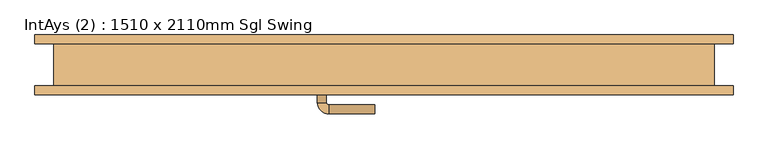
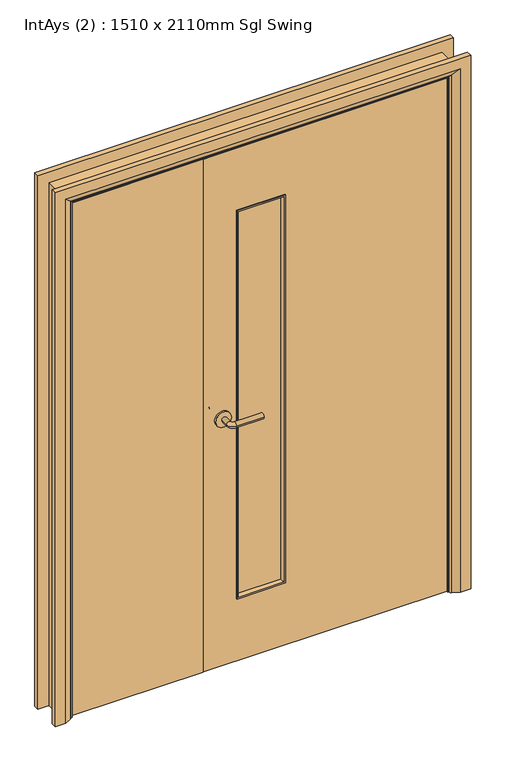
"""IFC4 building model written with IfcOpenShell, lengths in millimetres: door geometry, IntAys (2) : 1510 x 2110mm Sgl Swing."""

from ifc_helpers import new_model, si_unit, point, frame, frame_2d, origin, place, context, project, spatial, polyline, circle_curve, ellipse_curve, trimmed, segment, composite_curve, outline, extrude, faceted_brep, source, transform, mapped, element, save
from ifc_brep_helpers import plane_surface, cylinder_surface, revolved_surface, advanced_brep


def intays_2_1510_x_2110mm_sgl_swing_7badbe2f(model_context):
    return source(origin(), model_context, "Body", "SolidModel", [
        advanced_brep(
        [(88.5, -7.5, 1000.0), (108.5, -7.5, 1000.0), (88.5, 22.5, 1000.0), (108.5, 22.5, 1000.0), (113.5, 27.5, 1000.0), (113.5, 47.5, 1000.0), (218.5, 47.5, 1000.0), (218.5, 27.5, 1000.0)],
        [
            (0, 1, circle_curve(frame((98.5, -7.5, 1000.0), z_axis=(0.0, -1.0, 0.0), x_axis=(1.0, 0.0, 0.0)), 10.0)),
            (1, 0, circle_curve(frame((98.5, -7.5, 1000.0), z_axis=(0.0, -1.0, 0.0), x_axis=(1.0, 0.0, 0.0)), 10.0)),
            (0, 2),
            (2, 3, circle_curve(frame((98.5, 22.5, 1000.0), z_axis=(0.0, -1.0, 0.0), x_axis=(1.0, 0.0, 0.0)), 10.0)),
            (3, 1),
            (3, 2, circle_curve(frame((98.5, 22.5, 1000.0), z_axis=(0.0, -1.0, 0.0), x_axis=(1.0, 0.0, 0.0)), 10.0)),
            (4, 3, circle_curve(frame((113.5, 22.5, 1000.0), z_axis=(0.0, 0.0, 1.0), x_axis=(-1.0, 0.0, 0.0)), 5.0)),
            (2, 5, circle_curve(frame((113.5, 22.5, 1000.0), z_axis=(0.0, 0.0, -1.0), x_axis=(-1.0, 0.0, 0.0)), 25.0)),
            (5, 4, circle_curve(frame((113.5, 37.5, 1000.0), z_axis=(-1.0, 0.0, 0.0), x_axis=(0.0, -1.0, 0.0)), 10.0)),
            (4, 5, circle_curve(frame((113.5, 37.5, 1000.0), z_axis=(-1.0, 0.0, 0.0), x_axis=(0.0, -1.0, 0.0)), 10.0)),
            (6, 7, circle_curve(frame((218.5, 37.5, 1000.0), z_axis=(1.0, 0.0, 0.0), x_axis=(0.0, -1.0, 0.0)), 10.0)),
            (7, 6, circle_curve(frame((218.5, 37.5, 1000.0), z_axis=(1.0, 0.0, 0.0), x_axis=(0.0, -1.0, 0.0)), 10.0)),
            (5, 6),
            (7, 4),
        ],
        [
            plane_surface(frame((98.5, -7.5, 1000.0), z_axis=(0.0, -1.0, 0.0), x_axis=(0.0, 0.0, 1.0))),
            cylinder_surface(frame((98.5, -7.5, 1000.0), z_axis=(0.0, -1.0, 0.0), x_axis=(1.0, 0.0, 0.0)), 10.0),
            revolved_surface(trimmed(ellipse_curve(frame((98.5, 22.5, 1000.0), z_axis=(0.0, -1.0, 0.0), x_axis=(1.0, 0.0, 0.0)), 10.0, 10.0), [point((88.5, 22.5, 1000.0))], [point((108.5, 22.5, 1000.0))], True, "CARTESIAN"), (113.5, 22.5, 1000.0), (0.0, 0.0, -1.0)),
            revolved_surface(trimmed(ellipse_curve(frame((98.5, 22.5, 1000.0), z_axis=(0.0, -1.0, 0.0), x_axis=(1.0, 0.0, 0.0)), 10.0, 10.0), [point((108.5, 22.5, 1000.0))], [point((88.5, 22.5, 1000.0))], True, "CARTESIAN"), (113.5, 22.5, 1000.0), (0.0, 0.0, -1.0)),
            plane_surface(frame((218.5, 37.5, 1000.0), z_axis=(1.0, 0.0, 0.0), x_axis=(0.0, 0.0, 1.0))),
            cylinder_surface(frame((113.5, 37.5, 1000.0), z_axis=(-1.0, 0.0, 0.0), x_axis=(0.0, -1.0, 0.0)), 10.0),
        ],
        [
            (0, [[1, 2]]),
            (1, [[-1, 3, 4, 5]]),
            (1, [[-2, -5, 6, -3]]),
            (2, [[7, -4, 8, 9]]),
            (3, [[-8, -6, -7, 10]]),
            (4, [[11, 12]]),
            (5, [[-9, 13, -12, 14]]),
            (5, [[-10, -14, -11, -13]]),
        ],
    ),
        extrude(outline(composite_curve([segment(trimmed(circle_curve(frame_2d((1000.0, 96.0)), 30.0), [point((1000.0, 66.0))], [point((1000.0, 126.0))], False, "CARTESIAN"), True, "CONTINUOUS"), segment(trimmed(circle_curve(frame_2d((1000.0, 96.0)), 30.0), [point((1000.0, 126.0))], [point((1000.0, 66.0))], False, "CARTESIAN"), True, "CONTINUOUS")], self_intersect=False)), frame((0.0, -15.5, 0.0), z_axis=(0.0, 1.0, 0.0), x_axis=(0.0, 0.0, 1.0)), (0.0, 0.0, 1.0), 8.0),
        advanced_brep(
        [(88.5, -55.5, 1000.0), (108.5, -55.5, 1000.0), (108.5, -85.5, 1000.0), (88.5, -85.5, 1000.0), (113.5, -90.5, 1000.0), (113.5, -110.5, 1000.0), (218.5, -110.5, 1000.0), (218.5, -90.5, 1000.0)],
        [
            (0, 1, circle_curve(frame((98.5, -55.5, 1000.0), z_axis=(0.0, 1.0, 0.0), x_axis=(1.0, 0.0, 0.0)), 10.0)),
            (1, 0, circle_curve(frame((98.5, -55.5, 1000.0), z_axis=(0.0, 1.0, 0.0), x_axis=(1.0, 0.0, 0.0)), 10.0)),
            (1, 2),
            (2, 3, circle_curve(frame((98.5, -85.5, 1000.0), z_axis=(0.0, 1.0, 0.0), x_axis=(1.0, 0.0, 0.0)), 10.0)),
            (3, 0),
            (3, 2, circle_curve(frame((98.5, -85.5, 1000.0), z_axis=(0.0, 1.0, 0.0), x_axis=(1.0, 0.0, 0.0)), 10.0)),
            (4, 5, circle_curve(frame((113.5, -100.5, 1000.0), z_axis=(-1.0, 0.0, 0.0), x_axis=(0.0, 1.0, 0.0)), 10.0)),
            (5, 3, circle_curve(frame((113.5, -85.5, 1000.0), z_axis=(0.0, 0.0, -1.0), x_axis=(-1.0, 0.0, 0.0)), 25.0)),
            (2, 4, circle_curve(frame((113.5, -85.5, 1000.0), z_axis=(0.0, 0.0, 1.0), x_axis=(-1.0, 0.0, 0.0)), 5.0)),
            (5, 4, circle_curve(frame((113.5, -100.5, 1000.0), z_axis=(-1.0, 0.0, 0.0), x_axis=(0.0, 1.0, 0.0)), 10.0)),
            (6, 7, circle_curve(frame((218.5, -100.5, 1000.0), z_axis=(1.0, 0.0, 0.0), x_axis=(0.0, 1.0, 0.0)), 10.0)),
            (7, 6, circle_curve(frame((218.5, -100.5, 1000.0), z_axis=(1.0, 0.0, 0.0), x_axis=(0.0, 1.0, 0.0)), 10.0)),
            (4, 7),
            (6, 5),
        ],
        [
            plane_surface(frame((98.5, -55.5, 1000.0), z_axis=(0.0, 1.0, 0.0), x_axis=(0.0, 0.0, 1.0))),
            cylinder_surface(frame((98.5, -55.5, 1000.0), z_axis=(0.0, 1.0, 0.0), x_axis=(1.0, 0.0, 0.0)), 10.0),
            revolved_surface(trimmed(ellipse_curve(frame((98.5, -85.5, 1000.0), z_axis=(0.0, -1.0, 0.0), x_axis=(1.0, 0.0, 0.0)), 10.0, 10.0), [point((88.5, -85.5, 1000.0))], [point((108.5, -85.5, 1000.0))], True, "CARTESIAN"), (113.5, -85.5, 1000.0), (0.0, 0.0, -1.0)),
            revolved_surface(trimmed(ellipse_curve(frame((98.5, -85.5, 1000.0), z_axis=(0.0, -1.0, 0.0), x_axis=(1.0, 0.0, 0.0)), 10.0, 10.0), [point((108.5, -85.5, 1000.0))], [point((88.5, -85.5, 1000.0))], True, "CARTESIAN"), (113.5, -85.5, 1000.0), (0.0, 0.0, -1.0)),
            plane_surface(frame((218.5, -100.5, 1000.0), z_axis=(1.0, 0.0, 0.0), x_axis=(0.0, 0.0, 1.0))),
            cylinder_surface(frame((113.5, -100.5, 1000.0), z_axis=(-1.0, 0.0, 0.0), x_axis=(0.0, 1.0, 0.0)), 10.0),
        ],
        [
            (0, [[1, 2]]),
            (1, [[3, 4, 5, -2]]),
            (1, [[-5, 6, -3, -1]]),
            (2, [[7, 8, -4, 9]]),
            (3, [[10, -9, -6, -8]]),
            (4, [[11, 12]]),
            (5, [[13, -11, 14, -7]]),
            (5, [[-14, -12, -13, -10]]),
        ],
    ),
        extrude(outline(composite_curve([segment(trimmed(circle_curve(frame_2d((1000.0, 96.0)), 30.0), [point((1000.0, 66.0))], [point((1000.0, 126.0))], False, "CARTESIAN"), True, "CONTINUOUS"), segment(trimmed(circle_curve(frame_2d((1000.0, 96.0)), 30.0), [point((1000.0, 126.0))], [point((1000.0, 66.0))], False, "CARTESIAN"), True, "CONTINUOUS")], self_intersect=False)), frame((0.0, -55.5, 0.0), z_axis=(0.0, 1.0, 0.0), x_axis=(0.0, 0.0, 1.0)), (0.0, 0.0, 1.0), 8.0),
        extrude(outline(polyline([(2102.0, -508.0), (0.0, -508.0), (0.0, -476.0), (2070.0, -476.0), (2070.0, 954.0), (0.0, 954.0), (0.0, 986.0), (2102.0, 986.0), (2102.0, -508.0)])), frame((0.0, -47.5, 0.0), z_axis=(0.0, 1.0, 0.0), x_axis=(0.0, 0.0, 1.0)), (0.0, 0.0, 1.0), 95.0),
        advanced_brep(
        [(-551.0, 67.5, 0.0), (-511.0, 67.5, 0.0), (-485.0, 53.5, 0.0), (-481.0, 47.5, 0.0), (-551.0, 47.5, 0.0), (-551.0, 47.5, 2145.0), (-551.0, 67.5, 2145.0), (-481.0, 47.5, 2075.0), (959.0, 47.5, 2075.0), (959.0, 47.5, 0.0), (1029.0, 47.5, 0.0), (1029.0, 47.5, 2145.0), (-485.0, 53.5, 2079.0), (-511.0, 67.5, 2105.0), (1029.0, 67.5, 2145.0), (1029.0, 67.5, 0.0), (989.0, 67.5, 0.0), (989.0, 67.5, 2105.0), (963.0, 53.5, 0.0), (963.0, 53.5, 2079.0)],
        [
            (0, 1),
            (1, 2),
            (2, 3, circle_curve(frame((-489.0, 46.5, 0.0), z_axis=(0.0, 0.0, -1.0), x_axis=(-1.0, 0.0, 0.0)), 8.0622577)),
            (3, 4),
            (4, 0),
            (4, 5),
            (5, 6),
            (6, 0),
            (3, 7),
            (7, 8),
            (8, 9),
            (9, 10),
            (10, 11),
            (11, 5),
            (2, 12),
            (12, 7, ellipse_curve(frame((-489.0, 46.5, 2083.0), z_axis=(-0.7071067811865475, 0.0, -0.7071067811865475), x_axis=(0.7071067811865474, 0.0, -0.7071067811865476)), 11.4017543, 8.0622577)),
            (1, 13),
            (13, 12),
            (6, 14),
            (14, 15),
            (15, 16),
            (16, 17),
            (17, 13),
            (10, 15),
            (14, 11),
            (9, 18, circle_curve(frame((967.0, 46.5, 0.0), z_axis=(0.0, 0.0, -1.0), x_axis=(1.0, 0.0, 0.0)), 8.0622577)),
            (18, 16),
            (19, 18),
            (8, 19, ellipse_curve(frame((967.0, 46.5, 2083.0), z_axis=(0.7071067811865475, 0.0, -0.7071067811865475), x_axis=(0.7071067811865474, 0.0, 0.7071067811865476)), 11.4017543, 8.0622577)),
            (19, 17),
            (12, 19),
        ],
        [
            plane_surface(frame((-481.0, 47.5, 0.0), z_axis=(0.0, 0.0, -1.0), x_axis=(0.0, 1.0, 0.0))),
            plane_surface(frame((-551.0, 67.5, 0.0), z_axis=(-1.0, 0.0, 0.0), x_axis=(0.0, 0.0, 1.0))),
            plane_surface(frame((-551.0, 47.5, 0.0), z_axis=(0.0, -1.0, 0.0), x_axis=(0.0, 0.0, 1.0))),
            cylinder_surface(frame((-489.0, 46.5, 0.0), z_axis=(0.0, 0.0, -1.0), x_axis=(-1.0, 0.0, 0.0)), 8.0622577),
            plane_surface(frame((-485.0, 53.5, 0.0), z_axis=(0.4740998230350183, 0.8804710999221749, 0.0), x_axis=(0.0, 0.0, 1.0))),
            plane_surface(frame((-511.0, 67.5, 0.0), z_axis=(0.0, 1.0, 0.0), x_axis=(0.0, 0.0, 1.0))),
            plane_surface(frame((1029.0, 67.5, 2145.0), z_axis=(1.0, 0.0, 0.0), x_axis=(0.0, 0.0, -1.0))),
            plane_surface(frame((959.0, 47.5, 0.0), z_axis=(0.0, 0.0, -1.0), x_axis=(0.0, 1.0, 0.0))),
            cylinder_surface(frame((967.0, 46.5, 2075.0), z_axis=(0.0, 0.0, 1.0), x_axis=(1.0, 0.0, 0.0)), 8.0622577),
            plane_surface(frame((963.0, 53.5, 2079.0), z_axis=(-0.4740998230350183, 0.8804710999221749, 0.0), x_axis=(0.0, 0.0, -1.0))),
            plane_surface(frame((-551.0, 67.5, 2145.0), z_axis=(0.0, 0.0, 1.0), x_axis=(1.0, 0.0, 0.0))),
            cylinder_surface(frame((-481.0, 46.5, 2083.0), z_axis=(-1.0, 0.0, 0.0), x_axis=(0.0, 0.0, 1.0)), 8.0622577),
            plane_surface(frame((-485.0, 53.5, 2079.0), z_axis=(0.0, 0.8804710999221749, -0.4740998230350183), x_axis=(1.0, 0.0, 0.0))),
        ],
        [
            (0, [[1, 2, 3, 4, 5]]),
            (1, [[6, 7, 8, -5]]),
            (2, [[9, 10, 11, 12, 13, 14, -6, -4]]),
            (3, [[15, 16, -9, -3]]),
            (4, [[17, 18, -15, -2]]),
            (5, [[-8, 19, 20, 21, 22, 23, -17, -1]]),
            (6, [[-13, 24, -20, 25]]),
            (7, [[-24, -12, 26, 27, -21]]),
            (8, [[28, -26, -11, 29]]),
            (9, [[-22, -27, -28, 30]]),
            (10, [[-14, -25, -19, -7]]),
            (11, [[31, -29, -10, -16]]),
            (12, [[-23, -30, -31, -18]]),
        ],
    ),
        advanced_brep(
        [(1029.0, -67.5, 0.0), (989.0, -67.5, 0.0), (963.0, -53.5, 0.0), (959.0, -47.5, 0.0), (1029.0, -47.5, 0.0), (1029.0, -47.5, 2145.0), (1029.0, -67.5, 2145.0), (959.0, -47.5, 2075.0), (-481.0, -47.5, 2075.0), (-481.0, -47.5, 0.0), (-551.0, -47.5, 0.0), (-551.0, -47.5, 2145.0), (963.0, -53.5, 2079.0), (989.0, -67.5, 2105.0), (-551.0, -67.5, 2145.0), (-551.0, -67.5, 0.0), (-511.0, -67.5, 0.0), (-511.0, -67.5, 2105.0), (-485.0, -53.5, 0.0), (-485.0, -53.5, 2079.0)],
        [
            (0, 1),
            (1, 2),
            (2, 3, circle_curve(frame((967.0, -46.5, 0.0), z_axis=(0.0, 0.0, -1.0), x_axis=(1.0, 0.0, 0.0)), 8.0622577)),
            (3, 4),
            (4, 0),
            (4, 5),
            (5, 6),
            (6, 0),
            (3, 7),
            (7, 8),
            (8, 9),
            (9, 10),
            (10, 11),
            (11, 5),
            (2, 12),
            (12, 7, ellipse_curve(frame((967.0, -46.5, 2083.0), z_axis=(0.7071067811865475, 0.0, -0.7071067811865475), x_axis=(-0.7071067811865474, 0.0, -0.7071067811865476)), 11.4017543, 8.0622577)),
            (1, 13),
            (13, 12),
            (6, 14),
            (14, 15),
            (15, 16),
            (16, 17),
            (17, 13),
            (10, 15),
            (14, 11),
            (9, 18, circle_curve(frame((-489.0, -46.5, 0.0), z_axis=(0.0, 0.0, -1.0), x_axis=(-1.0, 0.0, 0.0)), 8.0622577)),
            (18, 16),
            (19, 18),
            (8, 19, ellipse_curve(frame((-489.0, -46.5, 2083.0), z_axis=(-0.7071067811865475, 0.0, -0.7071067811865475), x_axis=(-0.7071067811865474, 0.0, 0.7071067811865476)), 11.4017543, 8.0622577)),
            (19, 17),
            (12, 19),
        ],
        [
            plane_surface(frame((959.0, -47.5, 0.0), z_axis=(0.0, 0.0, -1.0), x_axis=(0.0, 1.0, 0.0))),
            plane_surface(frame((1029.0, -67.5, 0.0), z_axis=(1.0, 0.0, 0.0), x_axis=(0.0, 0.0, 1.0))),
            plane_surface(frame((1029.0, -47.5, 0.0), z_axis=(0.0, 1.0, 0.0), x_axis=(0.0, 0.0, 1.0))),
            cylinder_surface(frame((967.0, -46.5, 0.0), z_axis=(0.0, 0.0, -1.0), x_axis=(1.0, 0.0, 0.0)), 8.0622577),
            plane_surface(frame((963.0, -53.5, 0.0), z_axis=(-0.4740998230350126, -0.8804710999221779, 0.0), x_axis=(0.0, 0.0, 1.0))),
            plane_surface(frame((989.0, -67.5, 0.0), z_axis=(0.0, -1.0, 0.0), x_axis=(0.0, 0.0, 1.0))),
            plane_surface(frame((-551.0, -67.5, 2145.0), z_axis=(-1.0, 0.0, 0.0), x_axis=(0.0, 0.0, -1.0))),
            plane_surface(frame((-481.0, -47.5, 0.0), z_axis=(0.0, 0.0, -1.0), x_axis=(0.0, 1.0, 0.0))),
            cylinder_surface(frame((-489.0, -46.5, 2075.0), z_axis=(0.0, 0.0, 1.0), x_axis=(-1.0, 0.0, 0.0)), 8.0622577),
            plane_surface(frame((-485.0, -53.5, 2079.0), z_axis=(0.4740998230350183, -0.8804710999221749, 0.0), x_axis=(0.0, 0.0, -1.0))),
            plane_surface(frame((1029.0, -67.5, 2145.0), z_axis=(0.0, 0.0, 1.0), x_axis=(-1.0, 0.0, 0.0))),
            cylinder_surface(frame((959.0, -46.5, 2083.0), z_axis=(1.0, 0.0, 0.0), x_axis=(0.0, 0.0, 1.0)), 8.0622577),
            plane_surface(frame((963.0, -53.5, 2079.0), z_axis=(0.0, -0.8804710999221763, -0.4740998230350154), x_axis=(-1.0, 0.0, 0.0))),
        ],
        [
            (0, [[1, 2, 3, 4, 5]]),
            (1, [[6, 7, 8, -5]]),
            (2, [[9, 10, 11, 12, 13, 14, -6, -4]]),
            (3, [[15, 16, -9, -3]]),
            (4, [[17, 18, -15, -2]]),
            (5, [[-8, 19, 20, 21, 22, 23, -17, -1]]),
            (6, [[-13, 24, -20, 25]]),
            (7, [[-24, -12, 26, 27, -21]]),
            (8, [[28, -26, -11, 29]]),
            (9, [[-22, -27, -28, 30]]),
            (10, [[-14, -25, -19, -7]]),
            (11, [[31, -29, -10, -16]]),
            (12, [[-23, -30, -31, -18]]),
        ],
    ),
        faceted_brep([(-457.0, -12.5, 0.0), (-476.0, -12.5, 0.0), (-476.0, 19.5, 0.0), (-457.0, 19.5, 0.0), (-457.0, 19.5, 2051.0), (-457.0, -12.5, 2051.0), (-476.0, 19.5, 2070.0), (-476.0, -12.5, 2070.0), (935.0, -12.5, 0.0), (935.0, 19.5, 0.0), (954.0, 19.5, 0.0), (954.0, -12.5, 0.0), (935.0, -12.5, 2051.0), (954.0, -12.5, 2070.0), (954.0, 19.5, 2070.0), (935.0, 19.5, 2051.0)], [[[0, 1, 2, 3]], [[3, 4, 5, 0]], [[2, 6, 4, 3]], [[1, 7, 6, 2]], [[0, 5, 7, 1]], [[8, 9, 10, 11]], [[12, 8, 11, 13]], [[13, 11, 10, 14]], [[14, 10, 9, 15]], [[15, 9, 8, 12]], [[4, 15, 12, 5]], [[6, 14, 15, 4]], [[7, 13, 14, 6]], [[5, 12, 13, 7]]]),
        extrude(outline(polyline([(335.0, -25.5), (335.0, -37.5), (150.0, -37.5), (150.0, -25.5), (335.0, -25.5)])), frame((0.0, 0.0, 257.0), z_axis=(0.0, 0.0, 1.0), x_axis=(1.0, 0.0, 0.0)), (0.0, 0.0, 1.0), 1560.0),
        extrude(outline(polyline([(22.0, -15.5), (22.0, -47.5), (-473.0, -47.5), (-473.0, -15.5), (22.0, -15.5)])), frame((0.0, 0.0, 5.753223), z_axis=(0.0, 0.0, 1.0), x_axis=(1.0, 0.0, 0.0)), (0.0, 0.0, 1.0), 2061.246777),
        extrude(outline(polyline([(5.753223, 951.0), (2067.0, 951.0), (2067.0, 25.0), (5.753223, 25.0), (5.753223, 951.0)]), holes=[polyline([(1817.0, 150.0), (1817.0, 335.0), (257.0, 335.0), (257.0, 150.0), (1817.0, 150.0)])]), frame((0.0, -47.5, 0.0), z_axis=(0.0, 1.0, 0.0), x_axis=(0.0, 0.0, 1.0)), (0.0, 0.0, 1.0), 32.0),
        faceted_brep([(335.0, -12.5, 257.0), (335.0, -12.5, 1817.0), (335.0, -25.5, 1817.0), (335.0, -25.5, 257.0), (323.0, -25.5, 269.0), (323.0, -25.5, 1805.0), (329.0, -12.5, 1811.0), (329.0, -12.5, 263.0), (150.0, -12.5, 1817.0), (150.0, -25.5, 1817.0), (162.0, -25.5, 1805.0), (156.0, -12.5, 1811.0), (150.0, -12.5, 257.0), (150.0, -25.5, 257.0), (162.0, -25.5, 269.0), (156.0, -12.5, 263.0)], [[[0, 1, 2, 3]], [[4, 5, 6, 7]], [[1, 8, 9, 2]], [[5, 10, 11, 6]], [[8, 12, 13, 9]], [[10, 14, 15, 11]], [[3, 2, 9, 13], [5, 4, 14, 10]], [[12, 0, 3, 13]], [[1, 0, 12, 8], [7, 6, 11, 15]], [[14, 4, 7, 15]]]),
        faceted_brep([(150.0, -50.5, 257.0), (150.0, -50.5, 1817.0), (150.0, -37.5, 1817.0), (150.0, -37.5, 257.0), (162.0, -37.5, 269.0), (162.0, -37.5, 1805.0), (156.0, -50.5, 1811.0), (156.0, -50.5, 263.0), (335.0, -50.5, 1817.0), (335.0, -37.5, 1817.0), (323.0, -37.5, 1805.0), (329.0, -50.5, 1811.0), (335.0, -50.5, 257.0), (335.0, -37.5, 257.0), (323.0, -37.5, 269.0), (329.0, -50.5, 263.0)], [[[0, 1, 2, 3]], [[4, 5, 6, 7]], [[1, 8, 9, 2]], [[5, 10, 11, 6]], [[8, 12, 13, 9]], [[10, 14, 15, 11]], [[3, 2, 9, 13], [5, 4, 14, 10]], [[12, 0, 3, 13]], [[1, 0, 12, 8], [7, 6, 11, 15]], [[14, 4, 7, 15]]]),
    ])


if __name__ == "__main__":
    model = new_model("IFC4")
    model_context = context("Model", 3, world=origin())
    ifc_project = project(units=[si_unit("LENGTHUNIT", "METRE", prefix="MILLI")], contexts=[model_context])
    site = spatial("IfcSite", under=ifc_project)
    building = spatial("IfcBuilding", under=site)
    placement = place(None, origin())
    intays_2_1510_x_2110mm_sgl_swing_shape = intays_2_1510_x_2110mm_sgl_swing_7badbe2f(model_context)
    element("IfcDoor", 1, ObjectType="IntAys (2) : 1510 x 2110mm Sgl Swing", at=placement, inside=building, context=model_context, shape_type="MappedRepresentation", body=[
        mapped(intays_2_1510_x_2110mm_sgl_swing_shape, transform((0.0, 0.0, 0.0), x_axis=(1.0, 0.0, 0.0), y_axis=(0.0, 1.0, 0.0), z_axis=(0.0, 0.0, 1.0))),
    ])
    save(model, "model.ifc")

# Revit data of these elements
# Type "IntAys (2) : 1510 x 2110mm Sgl Swing"
#   Type Mark = "46"
#   Type Comments = "Internal Asymmetric"
#   Operation = "DoubleDoorSingleSwing"
#   Construction Type Id = "SGL"
#   Keynote = "L20"
#   Description = "Internal Asymmetric Door"
#   Analytic Construction = "Large single-glazed windows"
#   Visual Light Transmittance = 0.9
#   VisionPanel Width = 185 mm
#   Thickness = 32 mm
#   Stop Thickness = 19 mm
#   Stop Depth = 32 mm
#   Stile Top Rail = 250 mm
#   Stile Shutting = 125 mm
#   Stile Bottom Rail = 250 mm
#   Solar Heat Gain Coefficient = 0.86
#   Secondary Panel Width = 495 mm
#   Rough Width = 1510 mm
#   Rough Height = 2110 mm
#   Main Panel Width = 926 mm
#   Heat Transfer Coefficient (U) = 5.5617 W/(m²·K)
#   Handle Z Distance = 1000 mm
#   Handle X Distance = 75 mm
#   Handle Length = 350 mm
#   Frame Thickness = 32 mm
#   Door Panel Width = 926 mm
#   Door Panel Thickness = 32 mm
#   Height = 2110 mm
#   Door Panel Offset = 0 mm
#   Structural Tolerance = 8 mm
#   Tolerance = 3 mm
#   UnderCut = 7 mm
#   Width = 1510 mm
#   Door Panel Height = 2060 mm
#   Architrave Setback = 5 mm
#   Vis - Swing Single = yes
#   Vis - Swing Opposing = no
#   Vis - Swing Double = no
#   Vis - Stops = yes
#   Vis - Ironmongery = yes
#   Define Thermal Properties by = 1
#   Material Ironmongery = Door - Handle
#   Material Glass = Door - Glazing
#   Material Frame = Door - Frame/Mullion
#   Material Door = Door - Panel
#   Material Beading = Door - Panel
#   Material Architrave = Door - Architrave
#   Handle Style = element 261135
#   Function = (empty or 0)
#   Wall Closure = (empty or 0)
# Element 1 (IfcDoor, "IntAys (2) : 1510 x 2110mm Sgl Swing")
#   Materials on its faces: "Door - Panel", "Door - Architrave", "Door - Handle", "Door - Frame/Mullion", "Door - Glazing"
# Materials
#   "Door - Handle": class "Miscellaneous", colour RGB 0 0 0, transparency 0, Keynote = "P21"
#   "Door - Glazing": class "Miscellaneous", colour RGB 0 0 255, transparency 0.75
#   "Door - Frame/Mullion": class "Wood", colour RGB 212 179 113, transparency 0, Keynote = "L20"
#   "Door - Panel": class "Wood", colour RGB 210 159 95, transparency 0, Keynote = "L20"
#   "Door - Architrave": class "Wood", colour RGB 154 90 5, transparency 0, Keynote = "P20"
